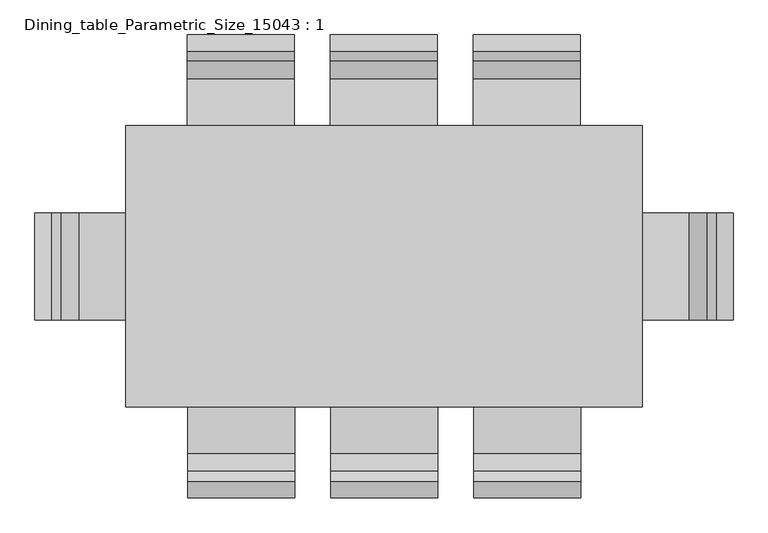
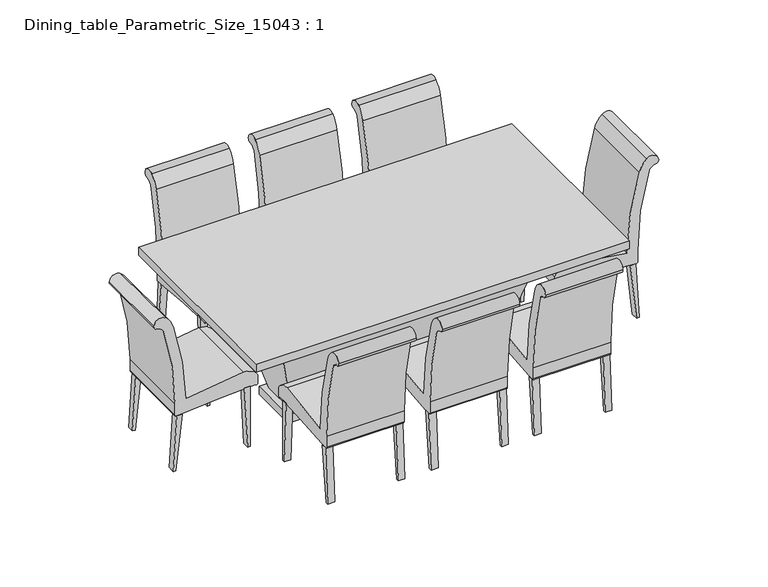
"""IFC4 building model written with IfcOpenShell, lengths in millimetres: furniture geometry, Dining_table_Parametric_Size_15043 : 1."""

from ifc_helpers import new_model, si_unit, point, frame, frame_2d, origin, place, context, project, spatial, polyline, circle_curve, trimmed, segment, composite_curve, outline, extrude, faceted_brep, source, transform, mapped, element, save


def dining_table_parametric_size_15043_1_d59548d5(model_context):
    return source(origin(), model_context, "Body", "SolidModel", [
        extrude(outline(polyline([(-435.6098174, 0.0), (-454.956828, 373.7391541), (-419.6521088, 373.7391541), (-419.6521088, 0.0), (-435.6098174, 0.0)])), frame((381.0, 0.0, 0.0), z_axis=(1.0, 0.0, 0.0), x_axis=(0.0, 1.0, 0.0)), (0.0, 0.0, 1.0), 38.1),
        extrude(outline(composite_curve([segment(polyline([(-852.8841698, 339.961294), (-821.1341698, 339.961294)]), True, "CONTINUOUS"), segment(trimmed(circle_curve(frame_2d((-4857.3831391, 601.3302132)), 4044.702641), [point((-821.1341698, 339.961294))], [point((-857.6304681, 0.0))], False, "CARTESIAN"), True, "CONTINUOUS"), segment(polyline([(-857.6304681, 0.0), (-873.6247987, 0.0)]), True, "CONTINUOUS"), segment(trimmed(circle_curve(frame_2d((-4939.427411, 418.6630455)), 4087.30102), [point((-873.6247987, 0.0))], [point((-852.8841698, 339.961294))], True, "CARTESIAN"), True, "CONTINUOUS")], self_intersect=False)), frame((382.3642545, 0.0, 0.0), z_axis=(1.0, 0.0, 0.0), x_axis=(0.0, 1.0, 0.0)), (0.0, 0.0, 1.0), 41.6791394),
        extrude(outline(polyline([(-433.0637156, 0.0), (-452.4107262, 373.7391541), (-417.106007, 373.7391541), (-417.106007, 0.0), (-433.0637156, 0.0)])), frame((800.1, 0.0, 0.0), z_axis=(1.0, 0.0, 0.0), x_axis=(0.0, 1.0, 0.0)), (0.0, 0.0, 1.0), 38.1),
        extrude(outline(composite_curve([segment(polyline([(-853.0334533, 339.961294), (-821.2834533, 339.961294)]), True, "CONTINUOUS"), segment(trimmed(circle_curve(frame_2d((-4857.5324226, 601.3302132)), 4044.702641), [point((-821.2834533, 339.961294))], [point((-857.7797517, 0.0))], False, "CARTESIAN"), True, "CONTINUOUS"), segment(polyline([(-857.7797517, 0.0), (-873.7740822, 0.0)]), True, "CONTINUOUS"), segment(trimmed(circle_curve(frame_2d((-4939.5766946, 418.6630455)), 4087.30102), [point((-873.7740822, 0.0))], [point((-853.0334533, 339.961294))], True, "CARTESIAN"), True, "CONTINUOUS")], self_intersect=False)), frame((800.1, 0.0, 0.0), z_axis=(1.0, 0.0, 0.0), x_axis=(0.0, 1.0, 0.0)), (0.0, 0.0, 1.0), 38.1),
        extrude(outline(composite_curve([segment(trimmed(circle_curve(frame_2d((-2597.9641625, 418.9322486)), 1733.8120537), [point((-864.1521088, 418.9322486))], [point((-931.3170473, 896.8356186))], True, "CARTESIAN"), True, "CONTINUOUS"), segment(trimmed(circle_curve(frame_2d((-979.3595379, 866.2613731)), 56.9461622), [point((-931.3170473, 896.8356186))], [point((-976.3560291, 923.1282732))], True, "CARTESIAN"), True, "CONTINUOUS"), segment(trimmed(circle_curve(frame_2d((-965.7723933, 942.5682988)), 22.134316), [point((-976.3560291, 923.1282732))], [point((-987.8415591, 944.2653155))], False, "CARTESIAN"), True, "CONTINUOUS"), segment(trimmed(circle_curve(frame_2d((-945.7630897, 941.029676)), 42.2026889), [point((-987.8415591, 944.2653155))], [point((-918.860453, 973.5460579))], False, "CARTESIAN"), True, "CONTINUOUS"), segment(trimmed(circle_curve(frame_2d((-1002.7657861, 872.1322861)), 131.6239265), [point((-918.860453, 973.5460579))], [point((-874.8340147, 903.0890285))], False, "CARTESIAN"), True, "CONTINUOUS"), segment(trimmed(circle_curve(frame_2d((-2637.1548845, 379.656989)), 1838.4112565), [point((-874.8340147, 903.0890285))], [point((-799.3387419, 426.4306353))], False, "CARTESIAN"), True, "CONTINUOUS"), segment(trimmed(circle_curve(frame_2d((-266.1478444, -2135.5006423)), 2616.8271636), [point((-799.3387419, 426.4306353))], [point((-459.7758211, 474.1530916))], False, "CARTESIAN"), True, "CONTINUOUS"), segment(trimmed(circle_curve(frame_2d((-453.2852539, 386.6753768)), 87.718174), [point((-459.7758211, 474.1530916))], [point((-375.6604678, 427.5271899))], False, "CARTESIAN"), True, "CONTINUOUS"), segment(polyline([(-375.6604678, 427.5271899), (-375.6604678, 371.8464813), (-380.1505959, 367.3563533), (-389.95219, 373.0153063)]), True, "CONTINUOUS"), segment(trimmed(circle_curve(frame_2d((-434.6347617, -793.4944233)), 1167.3651877), [point((-389.95219, 373.0153063))], [point((-600.0, 362.0988526))], True, "CARTESIAN"), True, "CONTINUOUS"), segment(trimmed(circle_curve(frame_2d((-928.0472905, 2654.5349591)), 2315.7889211), [point((-600.0, 362.0988526))], [point((-853.0334533, 339.961294))], False, "CARTESIAN"), True, "CONTINUOUS"), segment(trimmed(circle_curve(frame_2d((-854.8516896, 349.0822486)), 9.3004191), [point((-853.0334533, 339.961294))], [point((-864.1521088, 349.0822486))], False, "CARTESIAN"), True, "CONTINUOUS"), segment(polyline([(-864.1521088, 349.0822486), (-864.1521088, 418.9322486)]), True, "CONTINUOUS")], self_intersect=False)), frame((382.3642545, 0.0, 0.0), z_axis=(1.0, 0.0, 0.0), x_axis=(0.0, 1.0, 0.0)), (0.0, 0.0, 1.0), 455.8357455),
        extrude(outline(polyline([(435.6098174, 0.0), (419.6521088, 0.0), (419.6521088, 373.7391541), (454.956828, 373.7391541), (435.6098174, 0.0)])), frame((800.1, 0.0, 0.0), z_axis=(1.0, 0.0, 0.0), x_axis=(0.0, 1.0, 0.0)), (0.0, 0.0, 1.0), 38.1),
        extrude(outline(composite_curve([segment(trimmed(circle_curve(frame_2d((4939.427411, 418.6630455)), 4087.30102), [point((852.8841698, 339.961294))], [point((873.6247987, 0.0))], True, "CARTESIAN"), True, "CONTINUOUS"), segment(polyline([(873.6247987, 0.0), (857.6304681, 0.0)]), True, "CONTINUOUS"), segment(trimmed(circle_curve(frame_2d((4857.3831391, 601.3302132)), 4044.702641), [point((857.6304681, 0.0))], [point((821.1341698, 339.961294))], False, "CARTESIAN"), True, "CONTINUOUS"), segment(polyline([(821.1341698, 339.961294), (852.8841698, 339.961294)]), True, "CONTINUOUS")], self_intersect=False)), frame((795.1566061, 0.0, 0.0), z_axis=(1.0, 0.0, 0.0), x_axis=(0.0, 1.0, 0.0)), (0.0, 0.0, 1.0), 41.6791394),
        extrude(outline(polyline([(433.0637156, 0.0), (417.106007, 0.0), (417.106007, 373.7391541), (452.4107262, 373.7391541), (433.0637156, 0.0)])), frame((381.0, 0.0, 0.0), z_axis=(1.0, 0.0, 0.0), x_axis=(0.0, 1.0, 0.0)), (0.0, 0.0, 1.0), 38.1),
        extrude(outline(composite_curve([segment(trimmed(circle_curve(frame_2d((4939.5766946, 418.6630455)), 4087.30102), [point((853.0334533, 339.961294))], [point((873.7740822, 0.0))], True, "CARTESIAN"), True, "CONTINUOUS"), segment(polyline([(873.7740822, 0.0), (857.7797517, 0.0)]), True, "CONTINUOUS"), segment(trimmed(circle_curve(frame_2d((4857.5324226, 601.3302132)), 4044.702641), [point((857.7797517, 0.0))], [point((821.2834533, 339.961294))], False, "CARTESIAN"), True, "CONTINUOUS"), segment(polyline([(821.2834533, 339.961294), (853.0334533, 339.961294)]), True, "CONTINUOUS")], self_intersect=False)), frame((381.0, 0.0, 0.0), z_axis=(1.0, 0.0, 0.0), x_axis=(0.0, 1.0, 0.0)), (0.0, 0.0, 1.0), 38.1),
        extrude(outline(composite_curve([segment(polyline([(864.1521088, 418.9322486), (864.1521088, 349.0822486)]), True, "CONTINUOUS"), segment(trimmed(circle_curve(frame_2d((854.8516896, 349.0822486)), 9.3004191), [point((864.1521088, 349.0822486))], [point((853.0334533, 339.961294))], False, "CARTESIAN"), True, "CONTINUOUS"), segment(trimmed(circle_curve(frame_2d((928.0472905, 2654.5349591)), 2315.7889211), [point((853.0334533, 339.961294))], [point((600.0, 362.0988526))], False, "CARTESIAN"), True, "CONTINUOUS"), segment(trimmed(circle_curve(frame_2d((434.6347617, -793.4944233)), 1167.3651877), [point((600.0, 362.0988526))], [point((389.95219, 373.0153063))], True, "CARTESIAN"), True, "CONTINUOUS"), segment(polyline([(389.95219, 373.0153063), (380.1505959, 367.3563533), (375.6604678, 371.8464813), (375.6604678, 427.5271899)]), True, "CONTINUOUS"), segment(trimmed(circle_curve(frame_2d((453.2852539, 386.6753768)), 87.718174), [point((375.6604678, 427.5271899))], [point((459.7758211, 474.1530916))], False, "CARTESIAN"), True, "CONTINUOUS"), segment(trimmed(circle_curve(frame_2d((266.1478444, -2135.5006423)), 2616.8271636), [point((459.7758211, 474.1530916))], [point((799.3387419, 426.4306353))], False, "CARTESIAN"), True, "CONTINUOUS"), segment(trimmed(circle_curve(frame_2d((2637.1548845, 379.656989)), 1838.4112565), [point((799.3387419, 426.4306353))], [point((874.8340147, 903.0890285))], False, "CARTESIAN"), True, "CONTINUOUS"), segment(trimmed(circle_curve(frame_2d((1002.7657861, 872.1322861)), 131.6239265), [point((874.8340147, 903.0890285))], [point((918.860453, 973.5460579))], False, "CARTESIAN"), True, "CONTINUOUS"), segment(trimmed(circle_curve(frame_2d((945.7630897, 941.029676)), 42.2026889), [point((918.860453, 973.5460579))], [point((987.8415591, 944.2653155))], False, "CARTESIAN"), True, "CONTINUOUS"), segment(trimmed(circle_curve(frame_2d((965.7723933, 942.5682988)), 22.134316), [point((987.8415591, 944.2653155))], [point((976.3560291, 923.1282732))], False, "CARTESIAN"), True, "CONTINUOUS"), segment(trimmed(circle_curve(frame_2d((979.3595379, 866.2613731)), 56.9461622), [point((976.3560291, 923.1282732))], [point((931.3170473, 896.8356186))], True, "CARTESIAN"), True, "CONTINUOUS"), segment(trimmed(circle_curve(frame_2d((2597.9641625, 418.9322486)), 1733.8120537), [point((931.3170473, 896.8356186))], [point((864.1521088, 418.9322486))], True, "CARTESIAN"), True, "CONTINUOUS")], self_intersect=False)), frame((381.0, 0.0, 0.0), z_axis=(1.0, 0.0, 0.0), x_axis=(0.0, 1.0, 0.0)), (0.0, 0.0, 1.0), 455.8357455),
        extrude(outline(polyline([(-435.6098174, 0.0), (-454.956828, 373.7391541), (-419.6521088, 373.7391541), (-419.6521088, 0.0), (-435.6098174, 0.0)])), frame((-228.6, 0.0, 0.0), z_axis=(1.0, 0.0, 0.0), x_axis=(0.0, 1.0, 0.0)), (0.0, 0.0, 1.0), 38.1),
        extrude(outline(composite_curve([segment(polyline([(-852.8841698, 339.961294), (-821.1341698, 339.961294)]), True, "CONTINUOUS"), segment(trimmed(circle_curve(frame_2d((-4857.3831391, 601.3302132)), 4044.702641), [point((-821.1341698, 339.961294))], [point((-857.6304681, 0.0))], False, "CARTESIAN"), True, "CONTINUOUS"), segment(polyline([(-857.6304681, 0.0), (-873.6247987, 0.0)]), True, "CONTINUOUS"), segment(trimmed(circle_curve(frame_2d((-4939.427411, 418.6630455)), 4087.30102), [point((-873.6247987, 0.0))], [point((-852.8841698, 339.961294))], True, "CARTESIAN"), True, "CONTINUOUS")], self_intersect=False)), frame((-227.2357455, 0.0, 0.0), z_axis=(1.0, 0.0, 0.0), x_axis=(0.0, 1.0, 0.0)), (0.0, 0.0, 1.0), 41.6791394),
        extrude(outline(polyline([(-433.0637156, 0.0), (-452.4107262, 373.7391541), (-417.106007, 373.7391541), (-417.106007, 0.0), (-433.0637156, 0.0)])), frame((190.5, 0.0, 0.0), z_axis=(1.0, 0.0, 0.0), x_axis=(0.0, 1.0, 0.0)), (0.0, 0.0, 1.0), 38.1),
        extrude(outline(composite_curve([segment(polyline([(-853.0334533, 339.961294), (-821.2834533, 339.961294)]), True, "CONTINUOUS"), segment(trimmed(circle_curve(frame_2d((-4857.5324226, 601.3302132)), 4044.702641), [point((-821.2834533, 339.961294))], [point((-857.7797517, 0.0))], False, "CARTESIAN"), True, "CONTINUOUS"), segment(polyline([(-857.7797517, 0.0), (-873.7740822, 0.0)]), True, "CONTINUOUS"), segment(trimmed(circle_curve(frame_2d((-4939.5766946, 418.6630455)), 4087.30102), [point((-873.7740822, 0.0))], [point((-853.0334533, 339.961294))], True, "CARTESIAN"), True, "CONTINUOUS")], self_intersect=False)), frame((190.5, 0.0, 0.0), z_axis=(1.0, 0.0, 0.0), x_axis=(0.0, 1.0, 0.0)), (0.0, 0.0, 1.0), 38.1),
        extrude(outline(composite_curve([segment(trimmed(circle_curve(frame_2d((-2597.9641625, 418.9322486)), 1733.8120537), [point((-864.1521088, 418.9322486))], [point((-931.3170473, 896.8356186))], True, "CARTESIAN"), True, "CONTINUOUS"), segment(trimmed(circle_curve(frame_2d((-979.3595379, 866.2613731)), 56.9461622), [point((-931.3170473, 896.8356186))], [point((-976.3560291, 923.1282732))], True, "CARTESIAN"), True, "CONTINUOUS"), segment(trimmed(circle_curve(frame_2d((-965.7723933, 942.5682988)), 22.134316), [point((-976.3560291, 923.1282732))], [point((-987.8415591, 944.2653155))], False, "CARTESIAN"), True, "CONTINUOUS"), segment(trimmed(circle_curve(frame_2d((-945.7630897, 941.029676)), 42.2026889), [point((-987.8415591, 944.2653155))], [point((-918.860453, 973.5460579))], False, "CARTESIAN"), True, "CONTINUOUS"), segment(trimmed(circle_curve(frame_2d((-1002.7657861, 872.1322861)), 131.6239265), [point((-918.860453, 973.5460579))], [point((-874.8340147, 903.0890285))], False, "CARTESIAN"), True, "CONTINUOUS"), segment(trimmed(circle_curve(frame_2d((-2637.1548845, 379.656989)), 1838.4112565), [point((-874.8340147, 903.0890285))], [point((-799.3387419, 426.4306353))], False, "CARTESIAN"), True, "CONTINUOUS"), segment(trimmed(circle_curve(frame_2d((-266.1478444, -2135.5006423)), 2616.8271636), [point((-799.3387419, 426.4306353))], [point((-459.7758211, 474.1530916))], False, "CARTESIAN"), True, "CONTINUOUS"), segment(trimmed(circle_curve(frame_2d((-453.2852539, 386.6753768)), 87.718174), [point((-459.7758211, 474.1530916))], [point((-375.6604678, 427.5271899))], False, "CARTESIAN"), True, "CONTINUOUS"), segment(polyline([(-375.6604678, 427.5271899), (-375.6604678, 371.8464813), (-380.1505959, 367.3563533), (-389.95219, 373.0153063)]), True, "CONTINUOUS"), segment(trimmed(circle_curve(frame_2d((-434.6347617, -793.4944233)), 1167.3651877), [point((-389.95219, 373.0153063))], [point((-600.0, 362.0988526))], True, "CARTESIAN"), True, "CONTINUOUS"), segment(trimmed(circle_curve(frame_2d((-928.0472905, 2654.5349591)), 2315.7889211), [point((-600.0, 362.0988526))], [point((-853.0334533, 339.961294))], False, "CARTESIAN"), True, "CONTINUOUS"), segment(trimmed(circle_curve(frame_2d((-854.8516896, 349.0822486)), 9.3004191), [point((-853.0334533, 339.961294))], [point((-864.1521088, 349.0822486))], False, "CARTESIAN"), True, "CONTINUOUS"), segment(polyline([(-864.1521088, 349.0822486), (-864.1521088, 418.9322486)]), True, "CONTINUOUS")], self_intersect=False)), frame((-227.2357455, 0.0, 0.0), z_axis=(1.0, 0.0, 0.0), x_axis=(0.0, 1.0, 0.0)), (0.0, 0.0, 1.0), 455.8357455),
        extrude(outline(polyline([(-435.6098174, 0.0), (-454.956828, 373.7391541), (-419.6521088, 373.7391541), (-419.6521088, 0.0), (-435.6098174, 0.0)])), frame((-838.2, 0.0, 0.0), z_axis=(1.0, 0.0, 0.0), x_axis=(0.0, 1.0, 0.0)), (0.0, 0.0, 1.0), 38.1),
        extrude(outline(composite_curve([segment(polyline([(-852.8841698, 339.961294), (-821.1341698, 339.961294)]), True, "CONTINUOUS"), segment(trimmed(circle_curve(frame_2d((-4857.3831391, 601.3302132)), 4044.702641), [point((-821.1341698, 339.961294))], [point((-857.6304681, 0.0))], False, "CARTESIAN"), True, "CONTINUOUS"), segment(polyline([(-857.6304681, 0.0), (-873.6247987, 0.0)]), True, "CONTINUOUS"), segment(trimmed(circle_curve(frame_2d((-4939.427411, 418.6630455)), 4087.30102), [point((-873.6247987, 0.0))], [point((-852.8841698, 339.961294))], True, "CARTESIAN"), True, "CONTINUOUS")], self_intersect=False)), frame((-836.8357455, 0.0, 0.0), z_axis=(1.0, 0.0, 0.0), x_axis=(0.0, 1.0, 0.0)), (0.0, 0.0, 1.0), 41.6791394),
        extrude(outline(polyline([(-433.0637156, 0.0), (-452.4107262, 373.7391541), (-417.106007, 373.7391541), (-417.106007, 0.0), (-433.0637156, 0.0)])), frame((-419.1, 0.0, 0.0), z_axis=(1.0, 0.0, 0.0), x_axis=(0.0, 1.0, 0.0)), (0.0, 0.0, 1.0), 38.1),
        extrude(outline(composite_curve([segment(polyline([(-853.0334533, 339.961294), (-821.2834533, 339.961294)]), True, "CONTINUOUS"), segment(trimmed(circle_curve(frame_2d((-4857.5324226, 601.3302132)), 4044.702641), [point((-821.2834533, 339.961294))], [point((-857.7797517, 0.0))], False, "CARTESIAN"), True, "CONTINUOUS"), segment(polyline([(-857.7797517, 0.0), (-873.7740822, 0.0)]), True, "CONTINUOUS"), segment(trimmed(circle_curve(frame_2d((-4939.5766946, 418.6630455)), 4087.30102), [point((-873.7740822, 0.0))], [point((-853.0334533, 339.961294))], True, "CARTESIAN"), True, "CONTINUOUS")], self_intersect=False)), frame((-419.1, 0.0, 0.0), z_axis=(1.0, 0.0, 0.0), x_axis=(0.0, 1.0, 0.0)), (0.0, 0.0, 1.0), 38.1),
        extrude(outline(composite_curve([segment(trimmed(circle_curve(frame_2d((-2597.9641625, 418.9322486)), 1733.8120537), [point((-864.1521088, 418.9322486))], [point((-931.3170473, 896.8356186))], True, "CARTESIAN"), True, "CONTINUOUS"), segment(trimmed(circle_curve(frame_2d((-979.3595379, 866.2613731)), 56.9461622), [point((-931.3170473, 896.8356186))], [point((-976.3560291, 923.1282732))], True, "CARTESIAN"), True, "CONTINUOUS"), segment(trimmed(circle_curve(frame_2d((-965.7723933, 942.5682988)), 22.134316), [point((-976.3560291, 923.1282732))], [point((-987.8415591, 944.2653155))], False, "CARTESIAN"), True, "CONTINUOUS"), segment(trimmed(circle_curve(frame_2d((-945.7630897, 941.029676)), 42.2026889), [point((-987.8415591, 944.2653155))], [point((-918.860453, 973.5460579))], False, "CARTESIAN"), True, "CONTINUOUS"), segment(trimmed(circle_curve(frame_2d((-1002.7657861, 872.1322861)), 131.6239265), [point((-918.860453, 973.5460579))], [point((-874.8340147, 903.0890285))], False, "CARTESIAN"), True, "CONTINUOUS"), segment(trimmed(circle_curve(frame_2d((-2637.1548845, 379.656989)), 1838.4112565), [point((-874.8340147, 903.0890285))], [point((-799.3387419, 426.4306353))], False, "CARTESIAN"), True, "CONTINUOUS"), segment(trimmed(circle_curve(frame_2d((-266.1478444, -2135.5006423)), 2616.8271636), [point((-799.3387419, 426.4306353))], [point((-459.7758211, 474.1530916))], False, "CARTESIAN"), True, "CONTINUOUS"), segment(trimmed(circle_curve(frame_2d((-453.2852539, 386.6753768)), 87.718174), [point((-459.7758211, 474.1530916))], [point((-375.6604678, 427.5271899))], False, "CARTESIAN"), True, "CONTINUOUS"), segment(polyline([(-375.6604678, 427.5271899), (-375.6604678, 371.8464813), (-380.1505959, 367.3563533), (-389.95219, 373.0153063)]), True, "CONTINUOUS"), segment(trimmed(circle_curve(frame_2d((-434.6347617, -793.4944233)), 1167.3651877), [point((-389.95219, 373.0153063))], [point((-600.0, 362.0988526))], True, "CARTESIAN"), True, "CONTINUOUS"), segment(trimmed(circle_curve(frame_2d((-928.0472905, 2654.5349591)), 2315.7889211), [point((-600.0, 362.0988526))], [point((-853.0334533, 339.961294))], False, "CARTESIAN"), True, "CONTINUOUS"), segment(trimmed(circle_curve(frame_2d((-854.8516896, 349.0822486)), 9.3004191), [point((-853.0334533, 339.961294))], [point((-864.1521088, 349.0822486))], False, "CARTESIAN"), True, "CONTINUOUS"), segment(polyline([(-864.1521088, 349.0822486), (-864.1521088, 418.9322486)]), True, "CONTINUOUS")], self_intersect=False)), frame((-836.8357455, 0.0, 0.0), z_axis=(1.0, 0.0, 0.0), x_axis=(0.0, 1.0, 0.0)), (0.0, 0.0, 1.0), 455.8357455),
        extrude(outline(polyline([(435.6098174, 0.0), (419.6521088, 0.0), (419.6521088, 373.7391541), (454.956828, 373.7391541), (435.6098174, 0.0)])), frame((190.5, 0.0, 0.0), z_axis=(1.0, 0.0, 0.0), x_axis=(0.0, 1.0, 0.0)), (0.0, 0.0, 1.0), 38.1),
        extrude(outline(composite_curve([segment(trimmed(circle_curve(frame_2d((4939.427411, 418.6630455)), 4087.30102), [point((852.8841698, 339.961294))], [point((873.6247987, 0.0))], True, "CARTESIAN"), True, "CONTINUOUS"), segment(polyline([(873.6247987, 0.0), (857.6304681, 0.0)]), True, "CONTINUOUS"), segment(trimmed(circle_curve(frame_2d((4857.3831391, 601.3302132)), 4044.702641), [point((857.6304681, 0.0))], [point((821.1341698, 339.961294))], False, "CARTESIAN"), True, "CONTINUOUS"), segment(polyline([(821.1341698, 339.961294), (852.8841698, 339.961294)]), True, "CONTINUOUS")], self_intersect=False)), frame((185.5566061, 0.0, 0.0), z_axis=(1.0, 0.0, 0.0), x_axis=(0.0, 1.0, 0.0)), (0.0, 0.0, 1.0), 41.6791394),
        extrude(outline(polyline([(433.0637156, 0.0), (417.106007, 0.0), (417.106007, 373.7391541), (452.4107262, 373.7391541), (433.0637156, 0.0)])), frame((-228.6, 0.0, 0.0), z_axis=(1.0, 0.0, 0.0), x_axis=(0.0, 1.0, 0.0)), (0.0, 0.0, 1.0), 38.1),
        extrude(outline(composite_curve([segment(trimmed(circle_curve(frame_2d((4939.5766946, 418.6630455)), 4087.30102), [point((853.0334533, 339.961294))], [point((873.7740822, 0.0))], True, "CARTESIAN"), True, "CONTINUOUS"), segment(polyline([(873.7740822, 0.0), (857.7797517, 0.0)]), True, "CONTINUOUS"), segment(trimmed(circle_curve(frame_2d((4857.5324226, 601.3302132)), 4044.702641), [point((857.7797517, 0.0))], [point((821.2834533, 339.961294))], False, "CARTESIAN"), True, "CONTINUOUS"), segment(polyline([(821.2834533, 339.961294), (853.0334533, 339.961294)]), True, "CONTINUOUS")], self_intersect=False)), frame((-228.6, 0.0, 0.0), z_axis=(1.0, 0.0, 0.0), x_axis=(0.0, 1.0, 0.0)), (0.0, 0.0, 1.0), 38.1),
        extrude(outline(composite_curve([segment(polyline([(864.1521088, 418.9322486), (864.1521088, 349.0822486)]), True, "CONTINUOUS"), segment(trimmed(circle_curve(frame_2d((854.8516896, 349.0822486)), 9.3004191), [point((864.1521088, 349.0822486))], [point((853.0334533, 339.961294))], False, "CARTESIAN"), True, "CONTINUOUS"), segment(trimmed(circle_curve(frame_2d((928.0472905, 2654.5349591)), 2315.7889211), [point((853.0334533, 339.961294))], [point((600.0, 362.0988526))], False, "CARTESIAN"), True, "CONTINUOUS"), segment(trimmed(circle_curve(frame_2d((434.6347617, -793.4944233)), 1167.3651877), [point((600.0, 362.0988526))], [point((389.95219, 373.0153063))], True, "CARTESIAN"), True, "CONTINUOUS"), segment(polyline([(389.95219, 373.0153063), (380.1505959, 367.3563533), (375.6604678, 371.8464813), (375.6604678, 427.5271899)]), True, "CONTINUOUS"), segment(trimmed(circle_curve(frame_2d((453.2852539, 386.6753768)), 87.718174), [point((375.6604678, 427.5271899))], [point((459.7758211, 474.1530916))], False, "CARTESIAN"), True, "CONTINUOUS"), segment(trimmed(circle_curve(frame_2d((266.1478444, -2135.5006423)), 2616.8271636), [point((459.7758211, 474.1530916))], [point((799.3387419, 426.4306353))], False, "CARTESIAN"), True, "CONTINUOUS"), segment(trimmed(circle_curve(frame_2d((2637.1548845, 379.656989)), 1838.4112565), [point((799.3387419, 426.4306353))], [point((874.8340147, 903.0890285))], False, "CARTESIAN"), True, "CONTINUOUS"), segment(trimmed(circle_curve(frame_2d((1002.7657861, 872.1322861)), 131.6239265), [point((874.8340147, 903.0890285))], [point((918.860453, 973.5460579))], False, "CARTESIAN"), True, "CONTINUOUS"), segment(trimmed(circle_curve(frame_2d((945.7630897, 941.029676)), 42.2026889), [point((918.860453, 973.5460579))], [point((987.8415591, 944.2653155))], False, "CARTESIAN"), True, "CONTINUOUS"), segment(trimmed(circle_curve(frame_2d((965.7723933, 942.5682988)), 22.134316), [point((987.8415591, 944.2653155))], [point((976.3560291, 923.1282732))], False, "CARTESIAN"), True, "CONTINUOUS"), segment(trimmed(circle_curve(frame_2d((979.3595379, 866.2613731)), 56.9461622), [point((976.3560291, 923.1282732))], [point((931.3170473, 896.8356186))], True, "CARTESIAN"), True, "CONTINUOUS"), segment(trimmed(circle_curve(frame_2d((2597.9641625, 418.9322486)), 1733.8120537), [point((931.3170473, 896.8356186))], [point((864.1521088, 418.9322486))], True, "CARTESIAN"), True, "CONTINUOUS")], self_intersect=False)), frame((-228.6, 0.0, 0.0), z_axis=(1.0, 0.0, 0.0), x_axis=(0.0, 1.0, 0.0)), (0.0, 0.0, 1.0), 455.8357455),
        extrude(outline(polyline([(435.6098174, 0.0), (419.6521088, 0.0), (419.6521088, 373.7391541), (454.956828, 373.7391541), (435.6098174, 0.0)])), frame((-419.1, 0.0, 0.0), z_axis=(1.0, 0.0, 0.0), x_axis=(0.0, 1.0, 0.0)), (0.0, 0.0, 1.0), 38.1),
        extrude(outline(composite_curve([segment(trimmed(circle_curve(frame_2d((4939.427411, 418.6630455)), 4087.30102), [point((852.8841698, 339.961294))], [point((873.6247987, 0.0))], True, "CARTESIAN"), True, "CONTINUOUS"), segment(polyline([(873.6247987, 0.0), (857.6304681, 0.0)]), True, "CONTINUOUS"), segment(trimmed(circle_curve(frame_2d((4857.3831391, 601.3302132)), 4044.702641), [point((857.6304681, 0.0))], [point((821.1341698, 339.961294))], False, "CARTESIAN"), True, "CONTINUOUS"), segment(polyline([(821.1341698, 339.961294), (852.8841698, 339.961294)]), True, "CONTINUOUS")], self_intersect=False)), frame((-424.0433939, 0.0, 0.0), z_axis=(1.0, 0.0, 0.0), x_axis=(0.0, 1.0, 0.0)), (0.0, 0.0, 1.0), 41.6791394),
        extrude(outline(polyline([(433.0637156, 0.0), (417.106007, 0.0), (417.106007, 373.7391541), (452.4107262, 373.7391541), (433.0637156, 0.0)])), frame((-838.2, 0.0, 0.0), z_axis=(1.0, 0.0, 0.0), x_axis=(0.0, 1.0, 0.0)), (0.0, 0.0, 1.0), 38.1),
        extrude(outline(composite_curve([segment(trimmed(circle_curve(frame_2d((4939.5766946, 418.6630455)), 4087.30102), [point((853.0334533, 339.961294))], [point((873.7740822, 0.0))], True, "CARTESIAN"), True, "CONTINUOUS"), segment(polyline([(873.7740822, 0.0), (857.7797517, 0.0)]), True, "CONTINUOUS"), segment(trimmed(circle_curve(frame_2d((4857.5324226, 601.3302132)), 4044.702641), [point((857.7797517, 0.0))], [point((821.2834533, 339.961294))], False, "CARTESIAN"), True, "CONTINUOUS"), segment(polyline([(821.2834533, 339.961294), (853.0334533, 339.961294)]), True, "CONTINUOUS")], self_intersect=False)), frame((-838.2, 0.0, 0.0), z_axis=(1.0, 0.0, 0.0), x_axis=(0.0, 1.0, 0.0)), (0.0, 0.0, 1.0), 38.1),
        extrude(outline(composite_curve([segment(polyline([(864.1521088, 418.9322486), (864.1521088, 349.0822486)]), True, "CONTINUOUS"), segment(trimmed(circle_curve(frame_2d((854.8516896, 349.0822486)), 9.3004191), [point((864.1521088, 349.0822486))], [point((853.0334533, 339.961294))], False, "CARTESIAN"), True, "CONTINUOUS"), segment(trimmed(circle_curve(frame_2d((928.0472905, 2654.5349591)), 2315.7889211), [point((853.0334533, 339.961294))], [point((600.0, 362.0988526))], False, "CARTESIAN"), True, "CONTINUOUS"), segment(trimmed(circle_curve(frame_2d((434.6347617, -793.4944233)), 1167.3651877), [point((600.0, 362.0988526))], [point((389.95219, 373.0153063))], True, "CARTESIAN"), True, "CONTINUOUS"), segment(polyline([(389.95219, 373.0153063), (380.1505959, 367.3563533), (375.6604678, 371.8464813), (375.6604678, 427.5271899)]), True, "CONTINUOUS"), segment(trimmed(circle_curve(frame_2d((453.2852539, 386.6753768)), 87.718174), [point((375.6604678, 427.5271899))], [point((459.7758211, 474.1530916))], False, "CARTESIAN"), True, "CONTINUOUS"), segment(trimmed(circle_curve(frame_2d((266.1478444, -2135.5006423)), 2616.8271636), [point((459.7758211, 474.1530916))], [point((799.3387419, 426.4306353))], False, "CARTESIAN"), True, "CONTINUOUS"), segment(trimmed(circle_curve(frame_2d((2637.1548845, 379.656989)), 1838.4112565), [point((799.3387419, 426.4306353))], [point((874.8340147, 903.0890285))], False, "CARTESIAN"), True, "CONTINUOUS"), segment(trimmed(circle_curve(frame_2d((1002.7657861, 872.1322861)), 131.6239265), [point((874.8340147, 903.0890285))], [point((918.860453, 973.5460579))], False, "CARTESIAN"), True, "CONTINUOUS"), segment(trimmed(circle_curve(frame_2d((945.7630897, 941.029676)), 42.2026889), [point((918.860453, 973.5460579))], [point((987.8415591, 944.2653155))], False, "CARTESIAN"), True, "CONTINUOUS"), segment(trimmed(circle_curve(frame_2d((965.7723933, 942.5682988)), 22.134316), [point((987.8415591, 944.2653155))], [point((976.3560291, 923.1282732))], False, "CARTESIAN"), True, "CONTINUOUS"), segment(trimmed(circle_curve(frame_2d((979.3595379, 866.2613731)), 56.9461622), [point((976.3560291, 923.1282732))], [point((931.3170473, 896.8356186))], True, "CARTESIAN"), True, "CONTINUOUS"), segment(trimmed(circle_curve(frame_2d((2597.9641625, 418.9322486)), 1733.8120537), [point((931.3170473, 896.8356186))], [point((864.1521088, 418.9322486))], True, "CARTESIAN"), True, "CONTINUOUS")], self_intersect=False)), frame((-838.2, 0.0, 0.0), z_axis=(1.0, 0.0, 0.0), x_axis=(0.0, 1.0, 0.0)), (0.0, 0.0, 1.0), 455.8357455),
        extrude(outline(polyline([(0.0, -935.6098174), (0.0, -919.6521088), (373.7391541, -919.6521088), (373.7391541, -954.956828), (0.0, -935.6098174)])), frame((0.0, -228.6, 0.0), z_axis=(0.0, 1.0, 0.0), x_axis=(0.0, 0.0, 1.0)), (0.0, 0.0, 1.0), 38.1),
        extrude(outline(composite_curve([segment(trimmed(circle_curve(frame_2d((418.6630455, -5439.427411)), 4087.30102), [point((339.961294, -1352.8841698))], [point((0.0, -1373.6247987))], True, "CARTESIAN"), True, "CONTINUOUS"), segment(polyline([(0.0, -1373.6247987), (0.0, -1357.6304681)]), True, "CONTINUOUS"), segment(trimmed(circle_curve(frame_2d((601.3302132, -5357.3831391)), 4044.702641), [point((0.0, -1357.6304681))], [point((339.961294, -1321.1341698))], False, "CARTESIAN"), True, "CONTINUOUS"), segment(polyline([(339.961294, -1321.1341698), (339.961294, -1352.8841698)]), True, "CONTINUOUS")], self_intersect=False)), frame((0.0, -227.2357455, 0.0), z_axis=(0.0, 1.0, 0.0), x_axis=(0.0, 0.0, 1.0)), (0.0, 0.0, 1.0), 41.6791394),
        extrude(outline(polyline([(0.0, -933.0637156), (0.0, -917.106007), (373.7391541, -917.106007), (373.7391541, -952.4107262), (0.0, -933.0637156)])), frame((0.0, 190.5, 0.0), z_axis=(0.0, 1.0, 0.0), x_axis=(0.0, 0.0, 1.0)), (0.0, 0.0, 1.0), 38.1),
        extrude(outline(composite_curve([segment(trimmed(circle_curve(frame_2d((418.6630455, -5439.5766946)), 4087.30102), [point((339.961294, -1353.0334533))], [point((0.0, -1373.7740822))], True, "CARTESIAN"), True, "CONTINUOUS"), segment(polyline([(0.0, -1373.7740822), (0.0, -1357.7797517)]), True, "CONTINUOUS"), segment(trimmed(circle_curve(frame_2d((601.3302132, -5357.5324226)), 4044.702641), [point((0.0, -1357.7797517))], [point((339.961294, -1321.2834533))], False, "CARTESIAN"), True, "CONTINUOUS"), segment(polyline([(339.961294, -1321.2834533), (339.961294, -1353.0334533)]), True, "CONTINUOUS")], self_intersect=False)), frame((0.0, 190.5, 0.0), z_axis=(0.0, 1.0, 0.0), x_axis=(0.0, 0.0, 1.0)), (0.0, 0.0, 1.0), 38.1),
        extrude(outline(composite_curve([segment(polyline([(418.9322486, -1364.1521088), (349.0822486, -1364.1521088)]), True, "CONTINUOUS"), segment(trimmed(circle_curve(frame_2d((349.0822486, -1354.8516896)), 9.3004191), [point((349.0822486, -1364.1521088))], [point((339.961294, -1353.0334533))], False, "CARTESIAN"), True, "CONTINUOUS"), segment(trimmed(circle_curve(frame_2d((2654.5349591, -1428.0472905)), 2315.7889211), [point((339.961294, -1353.0334533))], [point((362.0988526, -1100.0))], False, "CARTESIAN"), True, "CONTINUOUS"), segment(trimmed(circle_curve(frame_2d((-793.4944233, -934.6347617)), 1167.3651877), [point((362.0988526, -1100.0))], [point((373.0153063, -889.95219))], True, "CARTESIAN"), True, "CONTINUOUS"), segment(polyline([(373.0153063, -889.95219), (367.3563533, -880.1505959), (371.8464813, -875.6604678), (427.5271899, -875.6604678)]), True, "CONTINUOUS"), segment(trimmed(circle_curve(frame_2d((386.6753768, -953.2852539)), 87.718174), [point((427.5271899, -875.6604678))], [point((474.1530916, -959.7758211))], False, "CARTESIAN"), True, "CONTINUOUS"), segment(trimmed(circle_curve(frame_2d((-2135.5006423, -766.1478444)), 2616.8271636), [point((474.1530916, -959.7758211))], [point((426.4306353, -1299.3387419))], False, "CARTESIAN"), True, "CONTINUOUS"), segment(trimmed(circle_curve(frame_2d((379.656989, -3137.1548845)), 1838.4112565), [point((426.4306353, -1299.3387419))], [point((903.0890285, -1374.8340147))], False, "CARTESIAN"), True, "CONTINUOUS"), segment(trimmed(circle_curve(frame_2d((872.1322861, -1502.7657861)), 131.6239265), [point((903.0890285, -1374.8340147))], [point((973.5460579, -1418.860453))], False, "CARTESIAN"), True, "CONTINUOUS"), segment(trimmed(circle_curve(frame_2d((941.029676, -1445.7630897)), 42.2026889), [point((973.5460579, -1418.860453))], [point((944.2653155, -1487.8415591))], False, "CARTESIAN"), True, "CONTINUOUS"), segment(trimmed(circle_curve(frame_2d((942.5682988, -1465.7723933)), 22.134316), [point((944.2653155, -1487.8415591))], [point((923.1282732, -1476.3560291))], False, "CARTESIAN"), True, "CONTINUOUS"), segment(trimmed(circle_curve(frame_2d((866.2613731, -1479.3595379)), 56.9461622), [point((923.1282732, -1476.3560291))], [point((896.8356186, -1431.3170473))], True, "CARTESIAN"), True, "CONTINUOUS"), segment(trimmed(circle_curve(frame_2d((418.9322486, -3097.9641625)), 1733.8120537), [point((896.8356186, -1431.3170473))], [point((418.9322486, -1364.1521088))], True, "CARTESIAN"), True, "CONTINUOUS")], self_intersect=False)), frame((0.0, -227.2357455, 0.0), z_axis=(0.0, 1.0, 0.0), x_axis=(0.0, 0.0, 1.0)), (0.0, 0.0, 1.0), 455.8357455),
        extrude(outline(polyline([(0.0, 935.6098174), (373.7391541, 954.956828), (373.7391541, 919.6521088), (0.0, 919.6521088), (0.0, 935.6098174)])), frame((0.0, -228.6, 0.0), z_axis=(0.0, 1.0, 0.0), x_axis=(0.0, 0.0, 1.0)), (0.0, 0.0, 1.0), 38.1),
        extrude(outline(composite_curve([segment(polyline([(339.961294, 1352.8841698), (339.961294, 1321.1341698)]), True, "CONTINUOUS"), segment(trimmed(circle_curve(frame_2d((601.3302132, 5357.3831391)), 4044.702641), [point((339.961294, 1321.1341698))], [point((0.0, 1357.6304681))], False, "CARTESIAN"), True, "CONTINUOUS"), segment(polyline([(0.0, 1357.6304681), (0.0, 1373.6247987)]), True, "CONTINUOUS"), segment(trimmed(circle_curve(frame_2d((418.6630455, 5439.427411)), 4087.30102), [point((0.0, 1373.6247987))], [point((339.961294, 1352.8841698))], True, "CARTESIAN"), True, "CONTINUOUS")], self_intersect=False)), frame((0.0, -227.2357455, 0.0), z_axis=(0.0, 1.0, 0.0), x_axis=(0.0, 0.0, 1.0)), (0.0, 0.0, 1.0), 41.6791394),
        extrude(outline(polyline([(0.0, 933.0637156), (373.7391541, 952.4107262), (373.7391541, 917.106007), (0.0, 917.106007), (0.0, 933.0637156)])), frame((0.0, 190.5, 0.0), z_axis=(0.0, 1.0, 0.0), x_axis=(0.0, 0.0, 1.0)), (0.0, 0.0, 1.0), 38.1),
        extrude(outline(composite_curve([segment(polyline([(339.961294, 1353.0334533), (339.961294, 1321.2834533)]), True, "CONTINUOUS"), segment(trimmed(circle_curve(frame_2d((601.3302132, 5357.5324226)), 4044.702641), [point((339.961294, 1321.2834533))], [point((0.0, 1357.7797517))], False, "CARTESIAN"), True, "CONTINUOUS"), segment(polyline([(0.0, 1357.7797517), (0.0, 1373.7740822)]), True, "CONTINUOUS"), segment(trimmed(circle_curve(frame_2d((418.6630455, 5439.5766946)), 4087.30102), [point((0.0, 1373.7740822))], [point((339.961294, 1353.0334533))], True, "CARTESIAN"), True, "CONTINUOUS")], self_intersect=False)), frame((0.0, 190.5, 0.0), z_axis=(0.0, 1.0, 0.0), x_axis=(0.0, 0.0, 1.0)), (0.0, 0.0, 1.0), 38.1),
        extrude(outline(composite_curve([segment(trimmed(circle_curve(frame_2d((418.9322486, 3097.9641625)), 1733.8120537), [point((418.9322486, 1364.1521088))], [point((896.8356186, 1431.3170473))], True, "CARTESIAN"), True, "CONTINUOUS"), segment(trimmed(circle_curve(frame_2d((866.2613731, 1479.3595379)), 56.9461622), [point((896.8356186, 1431.3170473))], [point((923.1282732, 1476.3560291))], True, "CARTESIAN"), True, "CONTINUOUS"), segment(trimmed(circle_curve(frame_2d((942.5682988, 1465.7723933)), 22.134316), [point((923.1282732, 1476.3560291))], [point((944.2653155, 1487.8415591))], False, "CARTESIAN"), True, "CONTINUOUS"), segment(trimmed(circle_curve(frame_2d((941.029676, 1445.7630897)), 42.2026889), [point((944.2653155, 1487.8415591))], [point((973.5460579, 1418.860453))], False, "CARTESIAN"), True, "CONTINUOUS"), segment(trimmed(circle_curve(frame_2d((872.1322861, 1502.7657861)), 131.6239265), [point((973.5460579, 1418.860453))], [point((903.0890285, 1374.8340147))], False, "CARTESIAN"), True, "CONTINUOUS"), segment(trimmed(circle_curve(frame_2d((379.656989, 3137.1548845)), 1838.4112565), [point((903.0890285, 1374.8340147))], [point((426.4306353, 1299.3387419))], False, "CARTESIAN"), True, "CONTINUOUS"), segment(trimmed(circle_curve(frame_2d((-2135.5006423, 766.1478444)), 2616.8271636), [point((426.4306353, 1299.3387419))], [point((474.1530916, 959.7758211))], False, "CARTESIAN"), True, "CONTINUOUS"), segment(trimmed(circle_curve(frame_2d((386.6753768, 953.2852539)), 87.718174), [point((474.1530916, 959.7758211))], [point((427.5271899, 875.6604678))], False, "CARTESIAN"), True, "CONTINUOUS"), segment(polyline([(427.5271899, 875.6604678), (371.8464813, 875.6604678), (367.3563533, 880.1505959), (373.0153063, 889.95219)]), True, "CONTINUOUS"), segment(trimmed(circle_curve(frame_2d((-793.4944233, 934.6347617)), 1167.3651877), [point((373.0153063, 889.95219))], [point((362.0988526, 1100.0))], True, "CARTESIAN"), True, "CONTINUOUS"), segment(trimmed(circle_curve(frame_2d((2654.5349591, 1428.0472905)), 2315.7889211), [point((362.0988526, 1100.0))], [point((339.961294, 1353.0334533))], False, "CARTESIAN"), True, "CONTINUOUS"), segment(trimmed(circle_curve(frame_2d((349.0822486, 1354.8516896)), 9.3004191), [point((339.961294, 1353.0334533))], [point((349.0822486, 1364.1521088))], False, "CARTESIAN"), True, "CONTINUOUS"), segment(polyline([(349.0822486, 1364.1521088), (418.9322486, 1364.1521088)]), True, "CONTINUOUS")], self_intersect=False)), frame((0.0, -227.2357455, 0.0), z_axis=(0.0, 1.0, 0.0), x_axis=(0.0, 0.0, 1.0)), (0.0, 0.0, 1.0), 455.8357455),
        faceted_brep([(-800.0, 300.0, 750.0), (-800.0, -300.0, 750.0), (800.0, -300.0, 750.0), (800.0, 300.0, 750.0), (650.0, 150.0, 0.0), (650.0, -150.0, 0.0), (-650.0, -150.0, 0.0), (-650.0, 150.0, 0.0), (-613.3333333, 113.3333333, 50.0), (-613.3333333, -113.3333333, 50.0), (613.3333333, -113.3333333, 50.0), (613.3333333, 113.3333333, 50.0), (650.0, 150.0, 50.0), (-650.0, 150.0, 50.0), (-650.0, -150.0, 50.0), (650.0, -150.0, 50.0)], [[[0, 1, 2, 3]], [[4, 5, 6, 7]], [[1, 0, 8, 9]], [[2, 1, 9, 10]], [[3, 2, 10, 11]], [[0, 3, 11, 8]], [[12, 13, 14, 15], [9, 8, 11, 10]], [[13, 12, 4, 7]], [[14, 13, 7, 6]], [[15, 14, 6, 5]], [[12, 15, 5, 4]]]),
        extrude(outline(polyline([(-1100.0, 600.0), (1100.0, 600.0), (1100.0, -600.0), (-1100.0, -600.0), (-1100.0, 600.0)])), frame((0.0, 0.0, 750.0), z_axis=(0.0, 0.0, 1.0), x_axis=(1.0, 0.0, 0.0)), (0.0, 0.0, 1.0), 50.0),
    ])


if __name__ == "__main__":
    model = new_model("IFC4")
    model_context = context("Model", 3, world=origin())
    ifc_project = project(units=[si_unit("LENGTHUNIT", "METRE", prefix="MILLI")], contexts=[model_context])
    site = spatial("IfcSite", under=ifc_project)
    building = spatial("IfcBuilding", under=site)
    placement = place(None, origin())
    dining_table_parametric_size_15043_1_shape = dining_table_parametric_size_15043_1_d59548d5(model_context)
    element("IfcFurniture", 1, ObjectType="Dining_table_Parametric_Size_15043 : 1", at=placement, inside=building, context=model_context, shape_type="MappedRepresentation", body=[
        mapped(dining_table_parametric_size_15043_1_shape, transform((0.0, 0.0, 0.0), x_axis=(1.0, 0.0, 0.0), y_axis=(0.0, 1.0, 0.0), z_axis=(0.0, 0.0, 1.0))),
    ])
    save(model, "model.ifc")

# Revit data of these elements
# Type "Dining_table_Parametric_Size_15043 : 1"
#   Width = 3' - 11.24409"
#   Length = 7' - 2.61417"
#   First Chair Position = 1' - 7.30709"
#   Chair Space = 2' - 0"
#   Number of Chairs = 3
#   Table Material = none
# Element 1 (IfcFurniture, "Dining_table_Parametric_Size_15043 : 1")
#   Materials on its faces: "Wood Frame", "Fabric"
# Materials
#   "Wood Frame": class "Unassigned", colour RGB 38 11 4, transparency 0, Comments = "Rendering appearance not upgraded "
#   "Fabric": class "Fabric", colour RGB 80 80 80, transparency 0
